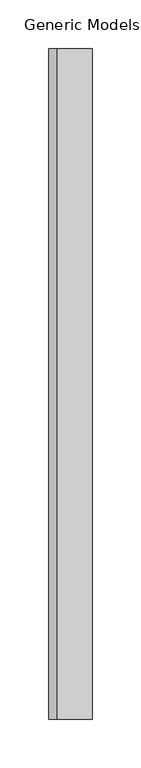
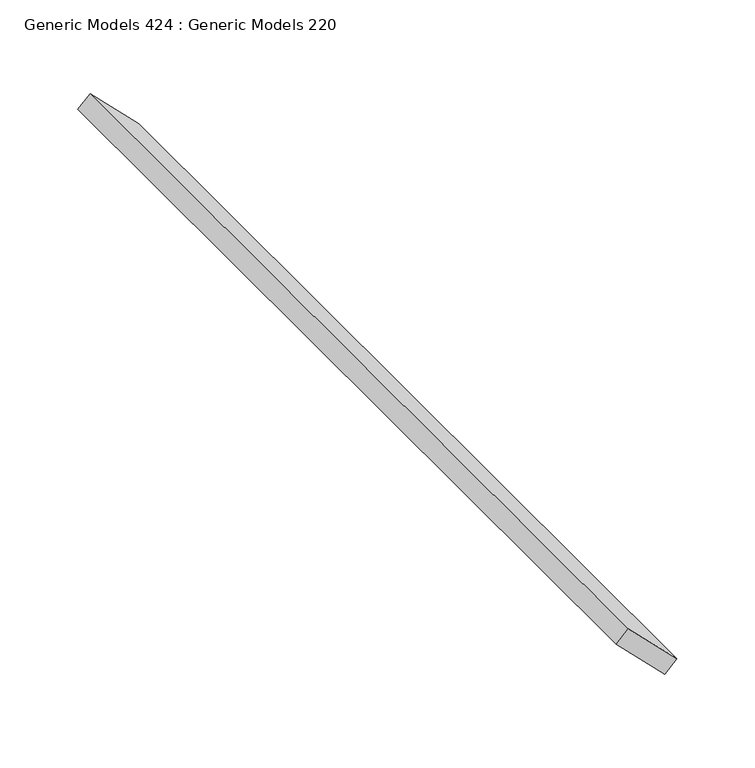
"""IFC4 building model written with IfcOpenShell, lengths in millimetres: proxy geometry, Generic Models 424 : Generic Models 220."""

import ifcopenshell
import ifcopenshell.guid

model = None  # the IFC model being written
_history = None  # IfcOwnerHistory: only IFC2X3 demands one
_inside = {}  # id of a spatial element -> (the spatial element, [elements in it])
_under = {}  # id of a project, library or spatial element -> (it, [spatial elements below it])
_declared = {}  # id of a project -> (the project, [libraries it declares])
_typed = {}  # id of a type object -> (the type object, [elements of that type])
_made_of = {}  # id of a material, layer set ... -> (it, [elements and type objects made of it])


def new_model(schema):
    """Start an empty IFC model of exactly this schema.

    Asked for "IFC4X3", IfcOpenShell would pick the latest addendum, in which some entities
    have other attributes; the version numbers below select the first issue.
    IFC2X3 requires an IfcOwnerHistory on every rooted entity: one is made here for all.
    """
    global model, _history
    if schema == "IFC4X3":
        model = ifcopenshell.file(schema_version=(4, 3, 0, 0))
    else:
        model = ifcopenshell.file(schema=schema)
    _inside.clear()
    _under.clear()
    _declared.clear()
    _typed.clear()
    _made_of.clear()
    _history = None
    if model.schema == "IFC2X3":
        org = make("IfcOrganization", Name="unknown")
        user = make(
            "IfcPersonAndOrganization",
            ThePerson=make("IfcPerson", FamilyName="unknown"),
            TheOrganization=org,
        )
        app = make(
            "IfcApplication",
            ApplicationDeveloper=org,
            Version="unknown",
            ApplicationFullName="unknown",
            ApplicationIdentifier="unknown",
        )
        _history = make(
            "IfcOwnerHistory",
            OwningUser=user,
            OwningApplication=app,
            ChangeAction="ADDED",
            CreationDate=0,
        )
    return model


def make(cls, **values):
    """One entity of the class cls with the attributes given. An attribute that is None is left unset."""
    return model.create_entity(
        cls, **{name: value for name, value in values.items() if value is not None}
    )


def rooted(cls, **values):
    """An entity with a GlobalId (a new one), such as an element, a storey or a relation."""
    return make(cls, GlobalId=ifcopenshell.guid.new(), OwnerHistory=_history, **values)


def si_unit(unit_type, name, prefix=None):
    """IfcSIUnit, for example si_unit("LENGTHUNIT", "METRE", prefix="MILLI")."""
    return make("IfcSIUnit", UnitType=unit_type, Prefix=prefix, Name=name)


def assignment(units):
    """IfcUnitAssignment: the units of a project."""
    return None if units is None else make("IfcUnitAssignment", Units=units)


def point(xyz):
    """IfcCartesianPoint."""
    return None if xyz is None else make("IfcCartesianPoint", Coordinates=xyz)


def direction(xyz):
    """IfcDirection."""
    return None if xyz is None else make("IfcDirection", DirectionRatios=xyz)


def frame(location, z_axis=None, x_axis=None):
    """IfcAxis2Placement3D, a coordinate frame: its origin and axes. An axis left out is left unset."""
    return make(
        "IfcAxis2Placement3D",
        Location=point(location),
        Axis=direction(z_axis),
        RefDirection=direction(x_axis),
    )


def origin():
    """The frame at (0, 0, 0) with its axes left unset."""
    return frame((0.0, 0.0, 0.0))


def place(relative_to, where):
    """IfcLocalPlacement: puts the frame where relative to a parent placement (None: the world)."""
    return make(
        "IfcLocalPlacement", PlacementRelTo=relative_to, RelativePlacement=where
    )


def context(
    kind, dimensions, precision=None, world=None, true_north=None, identifier=None
):
    """IfcGeometricRepresentationContext, for example the 3D "Model" context."""
    return make(
        "IfcGeometricRepresentationContext",
        ContextIdentifier=identifier,
        ContextType=kind,
        CoordinateSpaceDimension=dimensions,
        Precision=precision,
        WorldCoordinateSystem=world,
        TrueNorth=true_north,
    )


def project(units=None, contexts=None):
    """IfcProject with its units and contexts."""
    return rooted(
        "IfcProject",
        Name="project",
        RepresentationContexts=contexts,
        UnitsInContext=assignment(units),
    )


def spatial(cls, under=None, at=None, **own):
    """A site, building, storey or space (cls), placed at a placement, below another one or the project."""
    s = rooted(cls, ObjectPlacement=at, **own)
    if under is not None:
        _under.setdefault(under.id(), (under, []))[1].append(s)
    return s


def polyline(points):
    """IfcPolyline through the points."""
    return make("IfcPolyline", Points=[point(p) for p in points])


def outline(outer, holes=None, kind="AREA"):
    """IfcArbitraryClosedProfileDef: a profile drawn as a closed curve; with holes, ...WithVoids."""
    if holes is None:
        return make("IfcArbitraryClosedProfileDef", ProfileType=kind, OuterCurve=outer)
    return make(
        "IfcArbitraryProfileDefWithVoids",
        ProfileType=kind,
        OuterCurve=outer,
        InnerCurves=holes,
    )


def extrude(swept, where, along, depth):
    """IfcExtrudedAreaSolid: the profile swept, set in the frame where, extruded along a direction by depth."""
    return make(
        "IfcExtrudedAreaSolid",
        SweptArea=swept,
        Position=where,
        ExtrudedDirection=direction(along),
        Depth=depth,
    )


def shape(context_of_items, identifier, shape_type, items):
    """IfcShapeRepresentation: the items that make up one representation, for example the "Body"."""
    return make(
        "IfcShapeRepresentation",
        ContextOfItems=context_of_items,
        RepresentationIdentifier=identifier,
        RepresentationType=shape_type,
        Items=items,
    )


def source(mapping_origin, context_of_items, identifier, shape_type, items):
    """IfcRepresentationMap: a shape defined once, which mapped items show again and again."""
    return make(
        "IfcRepresentationMap",
        MappingOrigin=mapping_origin,
        MappedRepresentation=shape(context_of_items, identifier, shape_type, items),
    )


def transform(
    local_origin,
    x_axis=None,
    y_axis=None,
    z_axis=None,
    scale=None,
    scale2=None,
    scale3=None,
    uniform=True,
):
    """IfcCartesianTransformationOperator3D, or its non-uniform kind. x_axis, y_axis, z_axis: its Axis1, 2, 3."""
    if uniform:
        return make(
            "IfcCartesianTransformationOperator3D",
            Axis1=direction(x_axis),
            Axis2=direction(y_axis),
            LocalOrigin=point(local_origin),
            Scale=scale,
            Axis3=direction(z_axis),
        )
    return make(
        "IfcCartesianTransformationOperator3DnonUniform",
        Axis1=direction(x_axis),
        Axis2=direction(y_axis),
        LocalOrigin=point(local_origin),
        Scale=scale,
        Axis3=direction(z_axis),
        Scale2=scale2,
        Scale3=scale3,
    )


def mapped(mapping_source, mapping_target):
    """IfcMappedItem: shows the shape of a source again, moved by a transform."""
    return make(
        "IfcMappedItem", MappingSource=mapping_source, MappingTarget=mapping_target
    )


def made_of(thing, what):
    """Note that an element or type object is made of a material, layer set ...; save() writes the relation."""
    if what is not None:
        _made_of.setdefault(what.id(), (what, []))[1].append(thing)
    return thing


def element(
    cls,
    number,
    at=None,
    inside=None,
    cuts=None,
    type_object=None,
    material=None,
    context=None,
    identifier="Body",
    shape_type=None,
    held_by="IfcProductDefinitionShape",
    body=None,
    shapes=None,
    **own,
):
    """One element of the class cls, such as IfcWall. Its Tag is "e" and its number.

    at: its placement. inside: the storey or other place that contains it. cuts: it is an
    opening in that element (IfcRelVoidsElement). A single representation is given by context,
    identifier, shape_type and body (its items); several are given by shapes. held_by: the class
    of the entity that holds the representations. save() writes the other relations.
    """
    e = rooted(cls, Tag="e%d" % number, ObjectPlacement=at, **own)
    if body is not None:
        shapes = [shape(context, identifier, shape_type, body)]
    if shapes is not None:
        e.Representation = make(held_by, Representations=shapes)
    if inside is not None:
        _inside.setdefault(inside.id(), (inside, []))[1].append(e)
    if cuts is not None:
        rooted(
            "IfcRelVoidsElement", RelatingBuildingElement=cuts, RelatedOpeningElement=e
        )
    if type_object is not None:
        _typed.setdefault(type_object.id(), (type_object, []))[1].append(e)
    return made_of(e, material)


def aggregate(whole, parts):
    """IfcRelAggregates: a whole, such as a stair, and the parts it consists of."""
    return rooted("IfcRelAggregates", RelatingObject=whole, RelatedObjects=parts)


def save(model, path):
    """Write the relations noted so far, then the file.

    IfcRelAggregates (storeys below a building ...), IfcRelContainedInSpatialStructure (elements
    in a storey), IfcRelDefinesByType, IfcRelAssociatesMaterial and IfcRelDeclares: one each for
    every whole, place, type object, material and project.
    """
    for whole, parts in _under.values():
        aggregate(whole, parts)
    for where, things in _inside.values():
        rooted(
            "IfcRelContainedInSpatialStructure",
            RelatedElements=things,
            RelatingStructure=where,
        )
    for kind, things in _typed.values():
        rooted("IfcRelDefinesByType", RelatedObjects=things, RelatingType=kind)
    for what, things in _made_of.values():
        rooted("IfcRelAssociatesMaterial", RelatedObjects=things, RelatingMaterial=what)
    for by, libraries in _declared.values():
        rooted("IfcRelDeclares", RelatingContext=by, RelatedDefinitions=libraries)
    model.write(path)


def generic_models_424_generic_models_220_2f83cbba(model_context):
    return source(origin(), model_context, "Body", "SweptSolid", [
        extrude(outline(polyline([(0.0, -50.8), (0.0, 0.0), (690.8142348, 0.0), (690.8142348, -50.8), (0.0, -50.8)])), frame((-6899.085451, -4564.8872686, 128513.6762561), z_axis=(0.7071067811865582, 0.0, 0.7071067811865369), x_axis=(0.0, 1.0, 0.0)), (0.0, 0.0, 1.0), 12.7),
    ])


if __name__ == "__main__":
    model = new_model("IFC4")
    model_context = context("Model", 3, world=origin())
    ifc_project = project(units=[si_unit("LENGTHUNIT", "METRE", prefix="MILLI")], contexts=[model_context])
    site = spatial("IfcSite", under=ifc_project)
    building = spatial("IfcBuilding", under=site)
    placement = place(None, origin())
    generic_models_424_generic_models_220_shape = generic_models_424_generic_models_220_2f83cbba(model_context)
    element("IfcBuildingElementProxy", 1, Name="Generic Models 424 : Generic Models 220", ObjectType="Generic Models 424 : Generic Models 220", at=placement, inside=building, context=model_context, shape_type="MappedRepresentation", body=[
        mapped(generic_models_424_generic_models_220_shape, transform((0.0, 0.0, 0.0), x_axis=(1.0, 0.0, 0.0), y_axis=(0.0, 1.0, 0.0), z_axis=(0.0, 0.0, 1.0))),
    ])
    save(model, "model.ifc")

# Revit data of these elements
# Element 1 (IfcBuildingElementProxy, "Generic Models 424 : Generic Models 220")
#   Materials on its faces: "_WOOD TONE ALUMINUM EXTRUSION SLAT BY KNOTWOOD"
# Materials
#   "_WOOD TONE ALUMINUM EXTRUSION SLAT BY KNOTWOOD": class "Generic", colour RGB 177 130 114, transparency 0, Cost = 0
